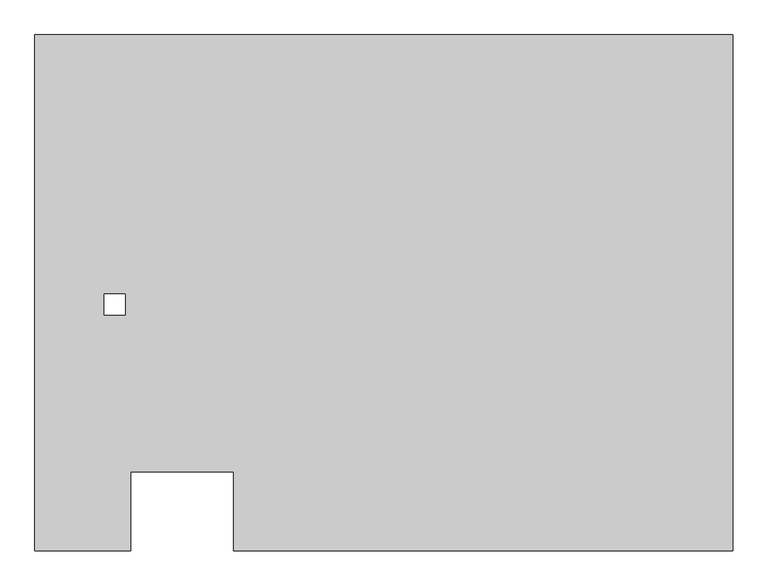
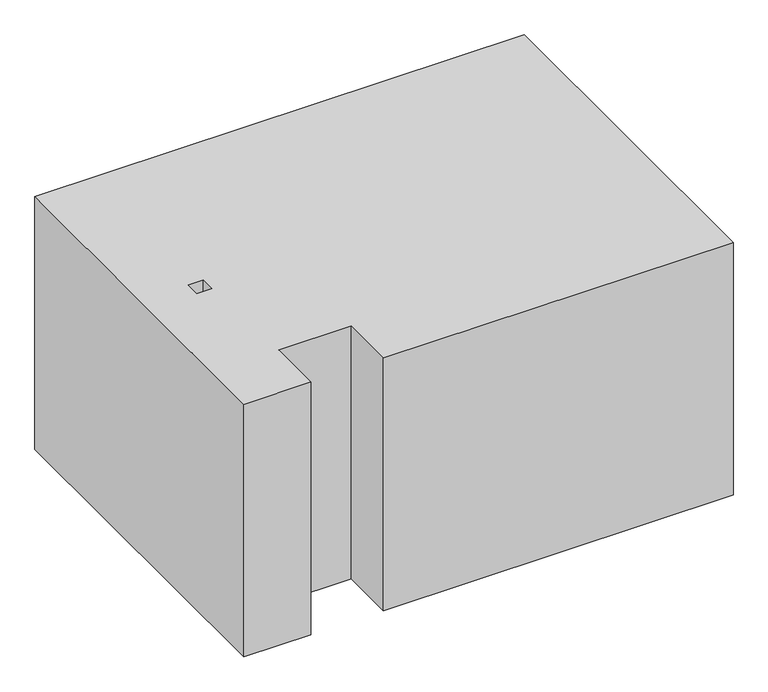
"""IFC4 building model written with IfcOpenShell, lengths in millimetres: proxy geometry, 0_3d_modell."""

from ifc_helpers import new_model, si_unit, origin, origin_with_axes, place, context, project, spatial, polyline, outline, extrude, source, transform, mapped, element, save


def generic_models_0598aa95(model_context):
    return source(origin(), model_context, "Body", "SweptSolid", [
        extrude(outline(polyline([(0.0, 3900.6204176), (5272.0, 3900.6204176), (5272.0, 0.0), (1502.0, 0.0), (1502.0, 600.0), (722.0, 600.0), (722.0, 0.0), (0.0, 0.0), (0.0, 3900.6204176)]), holes=[polyline([(522.0, 1943.3), (522.0, 1783.3), (682.0, 1783.3), (682.0, 1943.3), (522.0, 1943.3)])]), origin_with_axes(), (0.0, 0.0, 1.0), 2880.0),
    ])


if __name__ == "__main__":
    model = new_model("IFC4")
    model_context = context("Model", 3, world=origin())
    ifc_project = project(units=[si_unit("LENGTHUNIT", "METRE", prefix="MILLI")], contexts=[model_context])
    site = spatial("IfcSite", under=ifc_project)
    building = spatial("IfcBuilding", under=site)
    placement = place(None, origin())
    generic_models_shape = generic_models_0598aa95(model_context)
    element("IfcBuildingElementProxy", 1, Name="0_3d_modell", ObjectType="0_3d_modell", at=placement, inside=building, context=model_context, shape_type="MappedRepresentation", body=[
        mapped(generic_models_shape, transform((0.0, 0.0, 0.0), x_axis=(1.0, 0.0, 0.0), y_axis=(0.0, 1.0, 0.0), z_axis=(0.0, 0.0, 1.0))),
    ])
    save(model, "model.ifc")

# Revit data of these elements
# Element 1 (IfcBuildingElementProxy, "0_3d_modell")
#   Materials on its faces: "*1"
# Materials
#   "*1": class "Unassigned", colour RGB 175 175 175, transparency 0
